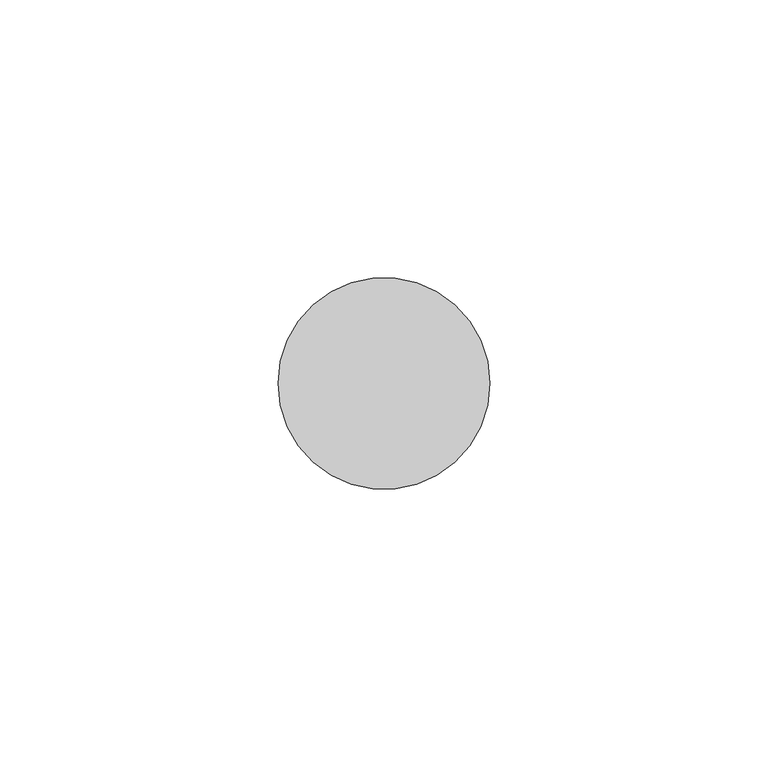
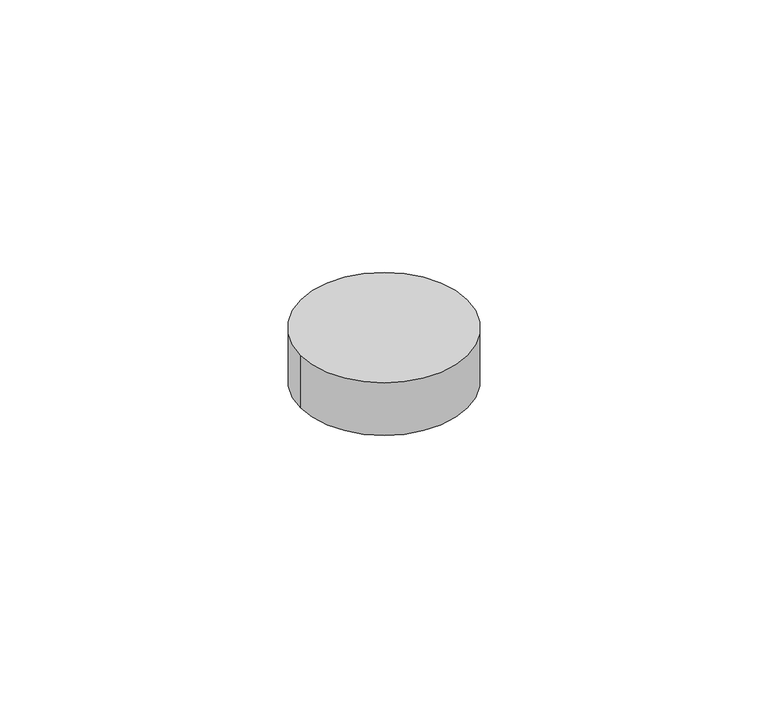
"""IFC4 building model written with IfcOpenShell, lengths in millimetres: proxy geometry, Bolt31:Bolt001:307947 : Bolt31:Bolt001:307947."""

from ifc_helpers import new_model, si_unit, point, frame, frame_2d, origin, place, context, project, spatial, circle_curve, trimmed, segment, composite_curve, outline, extrude, source, transform, mapped, element, save


def generic_models_5fc5945c(model_context):
    return source(origin(), model_context, "Body", "SweptSolid", [
        extrude(outline(composite_curve([segment(trimmed(circle_curve(frame_2d((12028.9793228, -1503.5124296)), 19.05), [point((12009.9293228, -1503.5124296))], [point((12048.0293228, -1503.5124296))], False, "CARTESIAN"), True, "CONTINUOUS"), segment(trimmed(circle_curve(frame_2d((12028.9793228, -1503.5124296)), 19.05), [point((12048.0293228, -1503.5124296))], [point((12009.9293228, -1503.5124296))], False, "CARTESIAN"), True, "CONTINUOUS")], self_intersect=False)), frame((0.0, 0.0, 40008.048), z_axis=(0.0, 0.0, 1.0), x_axis=(1.0, 0.0, 0.0)), (0.0, 0.0, 1.0), 12.7),
    ])


if __name__ == "__main__":
    model = new_model("IFC4")
    model_context = context("Model", 3, world=origin())
    ifc_project = project(units=[si_unit("LENGTHUNIT", "METRE", prefix="MILLI")], contexts=[model_context])
    site = spatial("IfcSite", under=ifc_project)
    building = spatial("IfcBuilding", under=site)
    placement = place(None, origin())
    generic_models_shape = generic_models_5fc5945c(model_context)
    element("IfcBuildingElementProxy", 1, Name="Bolt31:Bolt001:307947 : Bolt31:Bolt001:307947", ObjectType="Bolt31:Bolt001:307947 : Bolt31:Bolt001:307947", at=placement, inside=building, context=model_context, shape_type="MappedRepresentation", body=[
        mapped(generic_models_shape, transform((0.0, 0.0, 0.0), x_axis=(1.0, 0.0, 0.0), y_axis=(0.0, 1.0, 0.0), z_axis=(0.0, 0.0, 1.0))),
    ])
    save(model, "model.ifc")

# Revit data of these elements
# Type "Bolt31:Bolt001:307947 : Bolt31:Bolt001:307947"
#   NameOverride = "Bolt31:Bolt001:307947"
#   ObjectTypeOverride = "Bolt31:Bolt001"
#   Reference = "Bolt001"
#   Category = "Generic Models"
#   Tag = "307947"
# Element 1 (IfcBuildingElementProxy, "Bolt31:Bolt001:307947 : Bolt31:Bolt001:307947")
#   Materials on its faces: "BOLTS CONCEALED BY FLOOR FINISH"
# Materials
#   "BOLTS CONCEALED BY FLOOR FINISH": class "Unassigned", colour RGB 128 128 128, transparency 0
